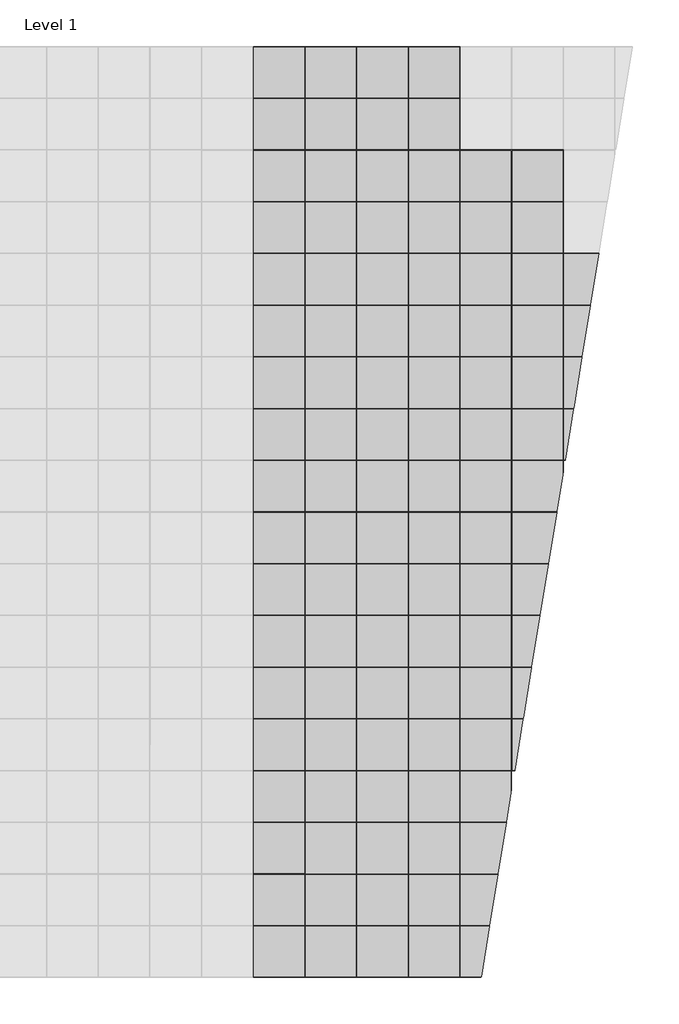
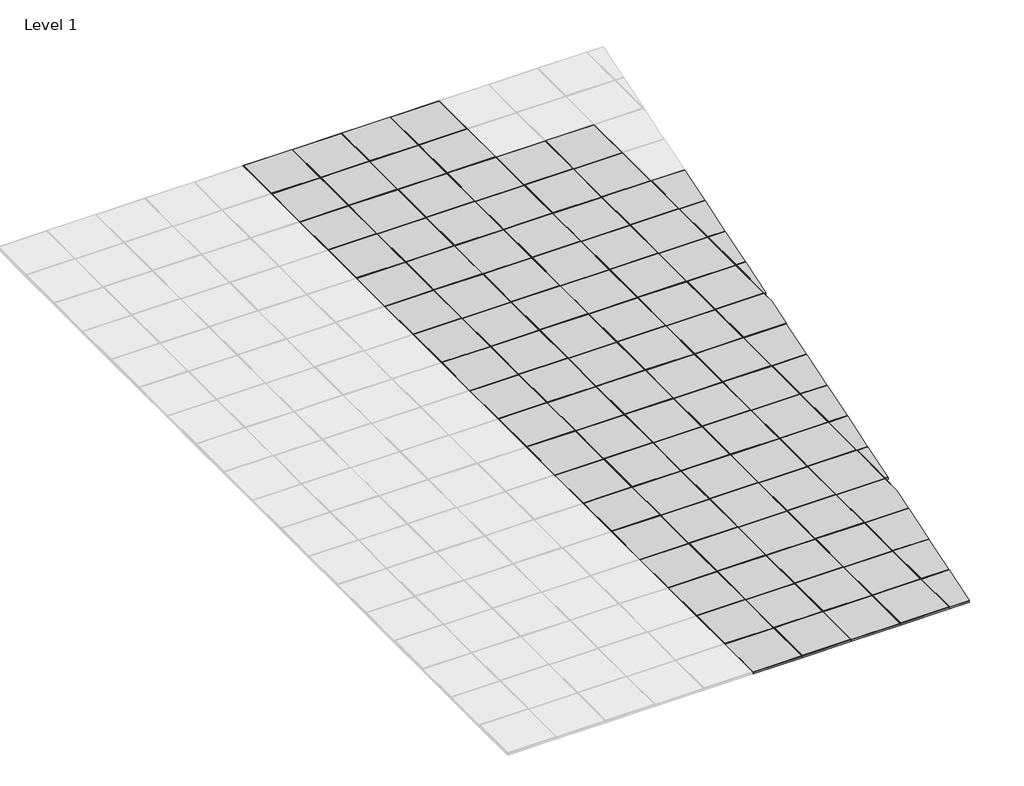
# One storey, part 2 of 18: 104 plates.
# Revit data of these elements (continued)
# Element 5 (IfcPlate, "00_CPA_tegel : Type 1") (continued)
#   Area = 0.248553 m²
#   Phase Created = New Construction
#   Materials on its faces: "20_voeg", "300_hardsteen_zwart"
# Element 6 (IfcPlate, "00_CPA_tegel : Type 1")
#   Area = 0.0109243 m²
#   Phase Created = New Construction
#   Materials on its faces: "20_voeg", "300_hardsteen_zwart"
# Element 7 (IfcPlate, "00_CPA_tegel : Type 1")
#   Area = 0.0846408 m²
#   Phase Created = New Construction
#   Materials on its faces: "20_voeg", "300_hardsteen_zwart"
# Element 8 (IfcPlate, "00_CPA_tegel : Type 1")
#   Area = 0.125286 m²
#   Phase Created = New Construction
#   Materials on its faces: "20_voeg", "300_hardsteen_zwart"
# Element 9 (IfcPlate, "00_CPA_tegel : Type 1")
#   Area = 0.0501228 m²
#   Phase Created = New Construction
#   Materials on its faces: "20_voeg", "300_hardsteen_zwart"
# Element 10 (IfcPlate, "00_CPA_tegel : Type 1")
#   Area = 0.0907683 m²
#   Phase Created = New Construction
#   Materials on its faces: "20_voeg", "300_hardsteen_zwart"
# Element 11 (IfcPlate, "00_CPA_tegel : Type 1")
#   Area = 0.131414 m²
#   Phase Created = New Construction
#   Materials on its faces: "20_voeg", "300_hardsteen_zwart"
# Element 12 (IfcPlate, "00_CPA_tegel : Type 1")
#   Area = 0.172059 m²
#   Phase Created = New Construction
#   Materials on its faces: "20_voeg", "300_hardsteen_zwart"
# Element 13 (IfcPlate, "00_CPA_tegel : Type 1")
#   Area = 0.212705 m²
#   Phase Created = New Construction
#   Materials on its faces: "20_voeg", "300_hardsteen_zwart"
# Element 14 (IfcPlate, "00_CPA_tegel : Type 1")
#   Area = 0.246456 m²
#   Phase Created = New Construction
#   Materials on its faces: "20_voeg", "300_hardsteen_zwart"
# Element 15 (IfcPlate, "00_CPA_tegel : Type 1")
#   Area = 0.0068939 m²
#   Phase Created = New Construction
#   Materials on its faces: "20_voeg", "300_hardsteen_zwart"
# Element 16 (IfcPlate, "00_CPA_tegel : Type 1")
#   Area = 0.0439958 m²
#   Phase Created = New Construction
#   Materials on its faces: "20_voeg", "300_hardsteen_zwart"
# Elements 17, 18, 19, 20, 21, 22, 23, 24, 25, 26, 27, 28, 29, 30, 31, 32, 33, 34, 35, 36, 37, 38, 39, 40, 41, 42, 43, 44, 45, 46, 47, 48, 49, 50, 51, 52, 53, 54, 55, 56, 57, 58, 59, 60, 61, 62, 63, 64, 65, 66, 67, 68, 69, 70, 71, 72, 73, 74, 75, 76, 77, 78, 79, 80, 81, 82, 83, 84, 85, 86, 87, 88, 89, 90, 91, 92, 93, 94, 95, 96, 97, 98, 99, 100, 101, 102, 103, 104 (IfcPlate, "00_CPA_tegel : Type 1")
#   Area = 0.25 m²
#   Phase Created = New Construction
#   Materials on its faces: "20_voeg", "300_hardsteen_zwart"
# Materials
#   "20_voeg": class "Concrete", colour RGB 86 86 86, transparency 0, Manufacturer = "RevitGG", URL = "www.revitgg.nl", Description = "zandcement, generiek materiaal", Cost = 0
#   "300_hardsteen_zwart": class "Generic", colour RGB 15 15 15, transparency 0, Description = "kalkzandsteen", Cost = 0
